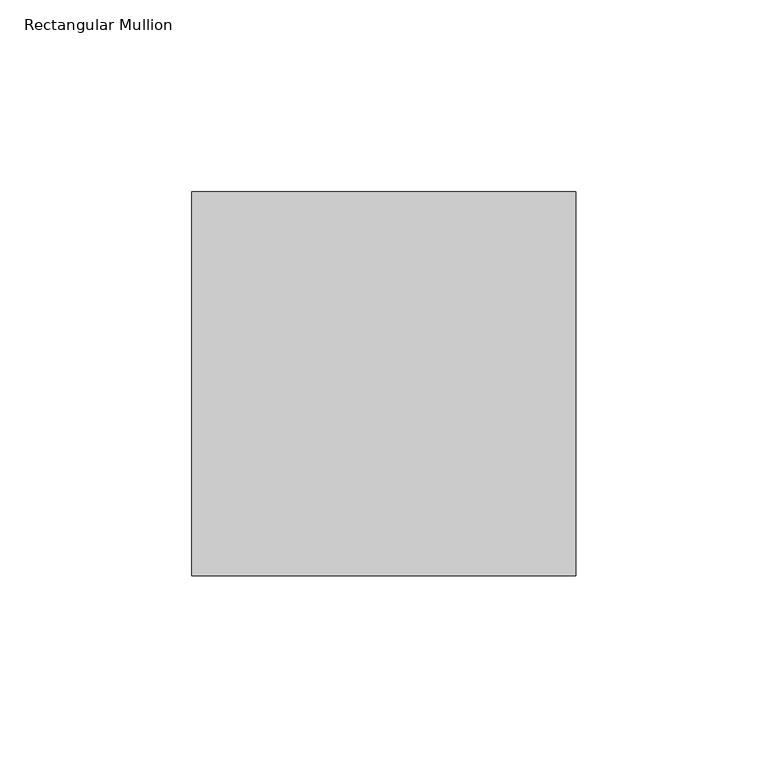
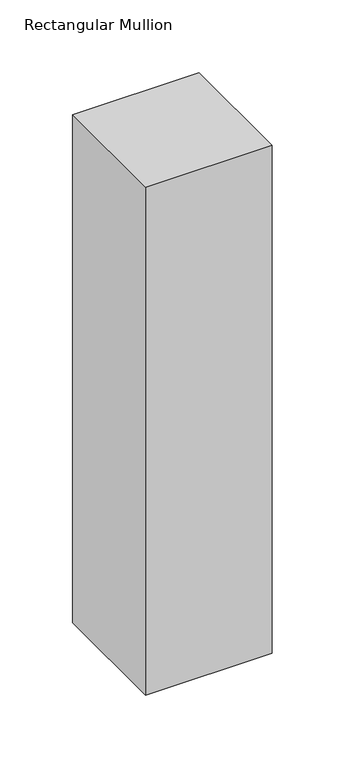
"""IFC4 building model written with IfcOpenShell, lengths in millimetres: member geometry, Rectangular Mullion : 알루미늄_Rectangular Cap_100 x100."""

import ifcopenshell
import ifcopenshell.guid

model = None  # the IFC model being written
_history = None  # IfcOwnerHistory: only IFC2X3 demands one
_inside = {}  # id of a spatial element -> (the spatial element, [elements in it])
_under = {}  # id of a project, library or spatial element -> (it, [spatial elements below it])
_declared = {}  # id of a project -> (the project, [libraries it declares])
_typed = {}  # id of a type object -> (the type object, [elements of that type])
_made_of = {}  # id of a material, layer set ... -> (it, [elements and type objects made of it])


def new_model(schema):
    """Start an empty IFC model of exactly this schema.

    Asked for "IFC4X3", IfcOpenShell would pick the latest addendum, in which some entities
    have other attributes; the version numbers below select the first issue.
    IFC2X3 requires an IfcOwnerHistory on every rooted entity: one is made here for all.
    """
    global model, _history
    if schema == "IFC4X3":
        model = ifcopenshell.file(schema_version=(4, 3, 0, 0))
    else:
        model = ifcopenshell.file(schema=schema)
    _inside.clear()
    _under.clear()
    _declared.clear()
    _typed.clear()
    _made_of.clear()
    _history = None
    if model.schema == "IFC2X3":
        org = make("IfcOrganization", Name="unknown")
        user = make(
            "IfcPersonAndOrganization",
            ThePerson=make("IfcPerson", FamilyName="unknown"),
            TheOrganization=org,
        )
        app = make(
            "IfcApplication",
            ApplicationDeveloper=org,
            Version="unknown",
            ApplicationFullName="unknown",
            ApplicationIdentifier="unknown",
        )
        _history = make(
            "IfcOwnerHistory",
            OwningUser=user,
            OwningApplication=app,
            ChangeAction="ADDED",
            CreationDate=0,
        )
    return model


def make(cls, **values):
    """One entity of the class cls with the attributes given. An attribute that is None is left unset."""
    return model.create_entity(
        cls, **{name: value for name, value in values.items() if value is not None}
    )


def rooted(cls, **values):
    """An entity with a GlobalId (a new one), such as an element, a storey or a relation."""
    return make(cls, GlobalId=ifcopenshell.guid.new(), OwnerHistory=_history, **values)


def si_unit(unit_type, name, prefix=None):
    """IfcSIUnit, for example si_unit("LENGTHUNIT", "METRE", prefix="MILLI")."""
    return make("IfcSIUnit", UnitType=unit_type, Prefix=prefix, Name=name)


def assignment(units):
    """IfcUnitAssignment: the units of a project."""
    return None if units is None else make("IfcUnitAssignment", Units=units)


def point(xyz):
    """IfcCartesianPoint."""
    return None if xyz is None else make("IfcCartesianPoint", Coordinates=xyz)


def direction(xyz):
    """IfcDirection."""
    return None if xyz is None else make("IfcDirection", DirectionRatios=xyz)


def frame(location, z_axis=None, x_axis=None):
    """IfcAxis2Placement3D, a coordinate frame: its origin and axes. An axis left out is left unset."""
    return make(
        "IfcAxis2Placement3D",
        Location=point(location),
        Axis=direction(z_axis),
        RefDirection=direction(x_axis),
    )


def origin():
    """The frame at (0, 0, 0) with its axes left unset."""
    return frame((0.0, 0.0, 0.0))


def place(relative_to, where):
    """IfcLocalPlacement: puts the frame where relative to a parent placement (None: the world)."""
    return make(
        "IfcLocalPlacement", PlacementRelTo=relative_to, RelativePlacement=where
    )


def context(
    kind, dimensions, precision=None, world=None, true_north=None, identifier=None
):
    """IfcGeometricRepresentationContext, for example the 3D "Model" context."""
    return make(
        "IfcGeometricRepresentationContext",
        ContextIdentifier=identifier,
        ContextType=kind,
        CoordinateSpaceDimension=dimensions,
        Precision=precision,
        WorldCoordinateSystem=world,
        TrueNorth=true_north,
    )


def project(units=None, contexts=None):
    """IfcProject with its units and contexts."""
    return rooted(
        "IfcProject",
        Name="project",
        RepresentationContexts=contexts,
        UnitsInContext=assignment(units),
    )


def spatial(cls, under=None, at=None, **own):
    """A site, building, storey or space (cls), placed at a placement, below another one or the project."""
    s = rooted(cls, ObjectPlacement=at, **own)
    if under is not None:
        _under.setdefault(under.id(), (under, []))[1].append(s)
    return s


def polyline(points):
    """IfcPolyline through the points."""
    return make("IfcPolyline", Points=[point(p) for p in points])


def outline(outer, holes=None, kind="AREA"):
    """IfcArbitraryClosedProfileDef: a profile drawn as a closed curve; with holes, ...WithVoids."""
    if holes is None:
        return make("IfcArbitraryClosedProfileDef", ProfileType=kind, OuterCurve=outer)
    return make(
        "IfcArbitraryProfileDefWithVoids",
        ProfileType=kind,
        OuterCurve=outer,
        InnerCurves=holes,
    )


def extrude(swept, where, along, depth):
    """IfcExtrudedAreaSolid: the profile swept, set in the frame where, extruded along a direction by depth."""
    return make(
        "IfcExtrudedAreaSolid",
        SweptArea=swept,
        Position=where,
        ExtrudedDirection=direction(along),
        Depth=depth,
    )


def shape(context_of_items, identifier, shape_type, items):
    """IfcShapeRepresentation: the items that make up one representation, for example the "Body"."""
    return make(
        "IfcShapeRepresentation",
        ContextOfItems=context_of_items,
        RepresentationIdentifier=identifier,
        RepresentationType=shape_type,
        Items=items,
    )


def source(mapping_origin, context_of_items, identifier, shape_type, items):
    """IfcRepresentationMap: a shape defined once, which mapped items show again and again."""
    return make(
        "IfcRepresentationMap",
        MappingOrigin=mapping_origin,
        MappedRepresentation=shape(context_of_items, identifier, shape_type, items),
    )


def transform(
    local_origin,
    x_axis=None,
    y_axis=None,
    z_axis=None,
    scale=None,
    scale2=None,
    scale3=None,
    uniform=True,
):
    """IfcCartesianTransformationOperator3D, or its non-uniform kind. x_axis, y_axis, z_axis: its Axis1, 2, 3."""
    if uniform:
        return make(
            "IfcCartesianTransformationOperator3D",
            Axis1=direction(x_axis),
            Axis2=direction(y_axis),
            LocalOrigin=point(local_origin),
            Scale=scale,
            Axis3=direction(z_axis),
        )
    return make(
        "IfcCartesianTransformationOperator3DnonUniform",
        Axis1=direction(x_axis),
        Axis2=direction(y_axis),
        LocalOrigin=point(local_origin),
        Scale=scale,
        Axis3=direction(z_axis),
        Scale2=scale2,
        Scale3=scale3,
    )


def mapped(mapping_source, mapping_target):
    """IfcMappedItem: shows the shape of a source again, moved by a transform."""
    return make(
        "IfcMappedItem", MappingSource=mapping_source, MappingTarget=mapping_target
    )


def made_of(thing, what):
    """Note that an element or type object is made of a material, layer set ...; save() writes the relation."""
    if what is not None:
        _made_of.setdefault(what.id(), (what, []))[1].append(thing)
    return thing


def element(
    cls,
    number,
    at=None,
    inside=None,
    cuts=None,
    type_object=None,
    material=None,
    context=None,
    identifier="Body",
    shape_type=None,
    held_by="IfcProductDefinitionShape",
    body=None,
    shapes=None,
    **own,
):
    """One element of the class cls, such as IfcWall. Its Tag is "e" and its number.

    at: its placement. inside: the storey or other place that contains it. cuts: it is an
    opening in that element (IfcRelVoidsElement). A single representation is given by context,
    identifier, shape_type and body (its items); several are given by shapes. held_by: the class
    of the entity that holds the representations. save() writes the other relations.
    """
    e = rooted(cls, Tag="e%d" % number, ObjectPlacement=at, **own)
    if body is not None:
        shapes = [shape(context, identifier, shape_type, body)]
    if shapes is not None:
        e.Representation = make(held_by, Representations=shapes)
    if inside is not None:
        _inside.setdefault(inside.id(), (inside, []))[1].append(e)
    if cuts is not None:
        rooted(
            "IfcRelVoidsElement", RelatingBuildingElement=cuts, RelatedOpeningElement=e
        )
    if type_object is not None:
        _typed.setdefault(type_object.id(), (type_object, []))[1].append(e)
    return made_of(e, material)


def aggregate(whole, parts):
    """IfcRelAggregates: a whole, such as a stair, and the parts it consists of."""
    return rooted("IfcRelAggregates", RelatingObject=whole, RelatedObjects=parts)


def save(model, path):
    """Write the relations noted so far, then the file.

    IfcRelAggregates (storeys below a building ...), IfcRelContainedInSpatialStructure (elements
    in a storey), IfcRelDefinesByType, IfcRelAssociatesMaterial and IfcRelDeclares: one each for
    every whole, place, type object, material and project.
    """
    for whole, parts in _under.values():
        aggregate(whole, parts)
    for where, things in _inside.values():
        rooted(
            "IfcRelContainedInSpatialStructure",
            RelatedElements=things,
            RelatingStructure=where,
        )
    for kind, things in _typed.values():
        rooted("IfcRelDefinesByType", RelatedObjects=things, RelatingType=kind)
    for what, things in _made_of.values():
        rooted("IfcRelAssociatesMaterial", RelatedObjects=things, RelatingMaterial=what)
    for by, libraries in _declared.values():
        rooted("IfcRelDeclares", RelatingContext=by, RelatedDefinitions=libraries)
    model.write(path)


def rectangular_mullion_bd602285(model_context):
    return source(origin(), model_context, "Body", "SweptSolid", [
        extrude(outline(polyline([(0.0, 50.0), (0.0, -50.0), (-100.0, -50.0), (-100.0, 50.0), (0.0, 50.0)])), frame((0.0, 0.0, -425.0), z_axis=(0.0, 0.0, 1.0), x_axis=(1.0, 0.0, 0.0)), (0.0, 0.0, 1.0), 425.0),
    ])


if __name__ == "__main__":
    model = new_model("IFC4")
    model_context = context("Model", 3, world=origin())
    ifc_project = project(units=[si_unit("LENGTHUNIT", "METRE", prefix="MILLI")], contexts=[model_context])
    site = spatial("IfcSite", under=ifc_project)
    building = spatial("IfcBuilding", under=site)
    placement = place(None, origin())
    rectangular_mullion_shape = rectangular_mullion_bd602285(model_context)
    element("IfcMember", 1, ObjectType="Rectangular Mullion : 알루미늄_Rectangular Cap_100 x100", at=placement, inside=building, context=model_context, shape_type="MappedRepresentation", body=[
        mapped(rectangular_mullion_shape, transform((0.0, 0.0, 0.0), x_axis=(1.0, 0.0, 0.0), y_axis=(0.0, 1.0, 0.0), z_axis=(0.0, 0.0, 1.0))),
    ])
    save(model, "model.ifc")

# Revit data of these elements
# Type "Rectangular Mullion : 알루미늄_Rectangular Cap_100 x100"
#   built-in parameter 1007304 = 0.328084 (stored number, unit not read)
#   built-in parameter 1007301 = 0.164042 (stored number, unit not read)
#   built-in parameter 1007300 = 0.164042 (stored number, unit not read)
# Element 1 (IfcMember, "Rectangular Mullion : 알루미늄_Rectangular Cap_100 x100")
#   Materials on its faces: "00_Metal_Stainless Steel"
# Materials
#   "00_Metal_Stainless Steel": class "Metal", colour RGB 148 148 148, transparency 0, Description = "Steel", Cost = 0
